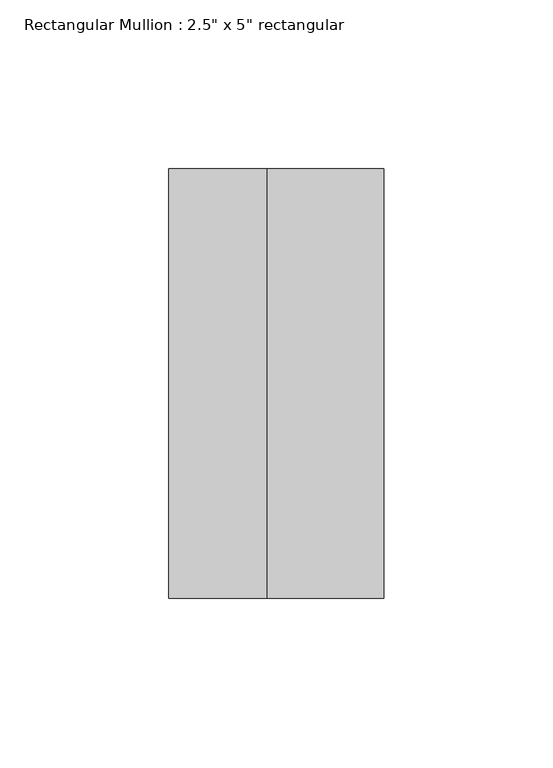
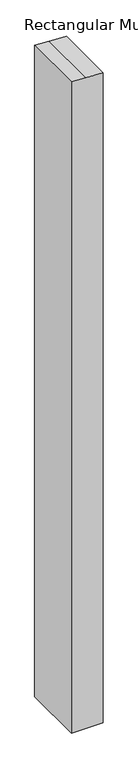
"""IFC4 building model written with IfcOpenShell, lengths in millimetres: member geometry."""

import ifcopenshell
import ifcopenshell.guid

model = None  # the IFC model being written
_history = None  # IfcOwnerHistory: only IFC2X3 demands one
_inside = {}  # id of a spatial element -> (the spatial element, [elements in it])
_under = {}  # id of a project, library or spatial element -> (it, [spatial elements below it])
_declared = {}  # id of a project -> (the project, [libraries it declares])
_typed = {}  # id of a type object -> (the type object, [elements of that type])
_made_of = {}  # id of a material, layer set ... -> (it, [elements and type objects made of it])


def new_model(schema):
    """Start an empty IFC model of exactly this schema.

    Asked for "IFC4X3", IfcOpenShell would pick the latest addendum, in which some entities
    have other attributes; the version numbers below select the first issue.
    IFC2X3 requires an IfcOwnerHistory on every rooted entity: one is made here for all.
    """
    global model, _history
    if schema == "IFC4X3":
        model = ifcopenshell.file(schema_version=(4, 3, 0, 0))
    else:
        model = ifcopenshell.file(schema=schema)
    _inside.clear()
    _under.clear()
    _declared.clear()
    _typed.clear()
    _made_of.clear()
    _history = None
    if model.schema == "IFC2X3":
        org = make("IfcOrganization", Name="unknown")
        user = make(
            "IfcPersonAndOrganization",
            ThePerson=make("IfcPerson", FamilyName="unknown"),
            TheOrganization=org,
        )
        app = make(
            "IfcApplication",
            ApplicationDeveloper=org,
            Version="unknown",
            ApplicationFullName="unknown",
            ApplicationIdentifier="unknown",
        )
        _history = make(
            "IfcOwnerHistory",
            OwningUser=user,
            OwningApplication=app,
            ChangeAction="ADDED",
            CreationDate=0,
        )
    return model


def make(cls, **values):
    """One entity of the class cls with the attributes given. An attribute that is None is left unset."""
    return model.create_entity(
        cls, **{name: value for name, value in values.items() if value is not None}
    )


def rooted(cls, **values):
    """An entity with a GlobalId (a new one), such as an element, a storey or a relation."""
    return make(cls, GlobalId=ifcopenshell.guid.new(), OwnerHistory=_history, **values)


def si_unit(unit_type, name, prefix=None):
    """IfcSIUnit, for example si_unit("LENGTHUNIT", "METRE", prefix="MILLI")."""
    return make("IfcSIUnit", UnitType=unit_type, Prefix=prefix, Name=name)


def assignment(units):
    """IfcUnitAssignment: the units of a project."""
    return None if units is None else make("IfcUnitAssignment", Units=units)


def point(xyz):
    """IfcCartesianPoint."""
    return None if xyz is None else make("IfcCartesianPoint", Coordinates=xyz)


def direction(xyz):
    """IfcDirection."""
    return None if xyz is None else make("IfcDirection", DirectionRatios=xyz)


def frame(location, z_axis=None, x_axis=None):
    """IfcAxis2Placement3D, a coordinate frame: its origin and axes. An axis left out is left unset."""
    return make(
        "IfcAxis2Placement3D",
        Location=point(location),
        Axis=direction(z_axis),
        RefDirection=direction(x_axis),
    )


def origin():
    """The frame at (0, 0, 0) with its axes left unset."""
    return frame((0.0, 0.0, 0.0))


def place(relative_to, where):
    """IfcLocalPlacement: puts the frame where relative to a parent placement (None: the world)."""
    return make(
        "IfcLocalPlacement", PlacementRelTo=relative_to, RelativePlacement=where
    )


def context(
    kind, dimensions, precision=None, world=None, true_north=None, identifier=None
):
    """IfcGeometricRepresentationContext, for example the 3D "Model" context."""
    return make(
        "IfcGeometricRepresentationContext",
        ContextIdentifier=identifier,
        ContextType=kind,
        CoordinateSpaceDimension=dimensions,
        Precision=precision,
        WorldCoordinateSystem=world,
        TrueNorth=true_north,
    )


def project(units=None, contexts=None):
    """IfcProject with its units and contexts."""
    return rooted(
        "IfcProject",
        Name="project",
        RepresentationContexts=contexts,
        UnitsInContext=assignment(units),
    )


def spatial(cls, under=None, at=None, **own):
    """A site, building, storey or space (cls), placed at a placement, below another one or the project."""
    s = rooted(cls, ObjectPlacement=at, **own)
    if under is not None:
        _under.setdefault(under.id(), (under, []))[1].append(s)
    return s


def polyline(points):
    """IfcPolyline through the points."""
    return make("IfcPolyline", Points=[point(p) for p in points])


def outline(outer, holes=None, kind="AREA"):
    """IfcArbitraryClosedProfileDef: a profile drawn as a closed curve; with holes, ...WithVoids."""
    if holes is None:
        return make("IfcArbitraryClosedProfileDef", ProfileType=kind, OuterCurve=outer)
    return make(
        "IfcArbitraryProfileDefWithVoids",
        ProfileType=kind,
        OuterCurve=outer,
        InnerCurves=holes,
    )


def extrude(swept, where, along, depth):
    """IfcExtrudedAreaSolid: the profile swept, set in the frame where, extruded along a direction by depth."""
    return make(
        "IfcExtrudedAreaSolid",
        SweptArea=swept,
        Position=where,
        ExtrudedDirection=direction(along),
        Depth=depth,
    )


def shape(context_of_items, identifier, shape_type, items):
    """IfcShapeRepresentation: the items that make up one representation, for example the "Body"."""
    return make(
        "IfcShapeRepresentation",
        ContextOfItems=context_of_items,
        RepresentationIdentifier=identifier,
        RepresentationType=shape_type,
        Items=items,
    )


def source(mapping_origin, context_of_items, identifier, shape_type, items):
    """IfcRepresentationMap: a shape defined once, which mapped items show again and again."""
    return make(
        "IfcRepresentationMap",
        MappingOrigin=mapping_origin,
        MappedRepresentation=shape(context_of_items, identifier, shape_type, items),
    )


def transform(
    local_origin,
    x_axis=None,
    y_axis=None,
    z_axis=None,
    scale=None,
    scale2=None,
    scale3=None,
    uniform=True,
):
    """IfcCartesianTransformationOperator3D, or its non-uniform kind. x_axis, y_axis, z_axis: its Axis1, 2, 3."""
    if uniform:
        return make(
            "IfcCartesianTransformationOperator3D",
            Axis1=direction(x_axis),
            Axis2=direction(y_axis),
            LocalOrigin=point(local_origin),
            Scale=scale,
            Axis3=direction(z_axis),
        )
    return make(
        "IfcCartesianTransformationOperator3DnonUniform",
        Axis1=direction(x_axis),
        Axis2=direction(y_axis),
        LocalOrigin=point(local_origin),
        Scale=scale,
        Axis3=direction(z_axis),
        Scale2=scale2,
        Scale3=scale3,
    )


def mapped(mapping_source, mapping_target):
    """IfcMappedItem: shows the shape of a source again, moved by a transform."""
    return make(
        "IfcMappedItem", MappingSource=mapping_source, MappingTarget=mapping_target
    )


def made_of(thing, what):
    """Note that an element or type object is made of a material, layer set ...; save() writes the relation."""
    if what is not None:
        _made_of.setdefault(what.id(), (what, []))[1].append(thing)
    return thing


def element(
    cls,
    number,
    at=None,
    inside=None,
    cuts=None,
    type_object=None,
    material=None,
    context=None,
    identifier="Body",
    shape_type=None,
    held_by="IfcProductDefinitionShape",
    body=None,
    shapes=None,
    **own,
):
    """One element of the class cls, such as IfcWall. Its Tag is "e" and its number.

    at: its placement. inside: the storey or other place that contains it. cuts: it is an
    opening in that element (IfcRelVoidsElement). A single representation is given by context,
    identifier, shape_type and body (its items); several are given by shapes. held_by: the class
    of the entity that holds the representations. save() writes the other relations.
    """
    e = rooted(cls, Tag="e%d" % number, ObjectPlacement=at, **own)
    if body is not None:
        shapes = [shape(context, identifier, shape_type, body)]
    if shapes is not None:
        e.Representation = make(held_by, Representations=shapes)
    if inside is not None:
        _inside.setdefault(inside.id(), (inside, []))[1].append(e)
    if cuts is not None:
        rooted(
            "IfcRelVoidsElement", RelatingBuildingElement=cuts, RelatedOpeningElement=e
        )
    if type_object is not None:
        _typed.setdefault(type_object.id(), (type_object, []))[1].append(e)
    return made_of(e, material)


def aggregate(whole, parts):
    """IfcRelAggregates: a whole, such as a stair, and the parts it consists of."""
    return rooted("IfcRelAggregates", RelatingObject=whole, RelatedObjects=parts)


def save(model, path):
    """Write the relations noted so far, then the file.

    IfcRelAggregates (storeys below a building ...), IfcRelContainedInSpatialStructure (elements
    in a storey), IfcRelDefinesByType, IfcRelAssociatesMaterial and IfcRelDeclares: one each for
    every whole, place, type object, material and project.
    """
    for whole, parts in _under.values():
        aggregate(whole, parts)
    for where, things in _inside.values():
        rooted(
            "IfcRelContainedInSpatialStructure",
            RelatedElements=things,
            RelatingStructure=where,
        )
    for kind, things in _typed.values():
        rooted("IfcRelDefinesByType", RelatedObjects=things, RelatingType=kind)
    for what, things in _made_of.values():
        rooted("IfcRelAssociatesMaterial", RelatedObjects=things, RelatingMaterial=what)
    for by, libraries in _declared.values():
        rooted("IfcRelDeclares", RelatingContext=by, RelatedDefinitions=libraries)
    model.write(path)


def member_2c70c373(model_context):
    return source(origin(), model_context, "Body", "SweptSolid", [
        extrude(outline(polyline([(-64.8775557, 31.75), (-63.4449853, -2.6426951), (-62.232569, -31.75), (-1437.7204901, -31.75), (-1437.7204901, 31.75), (-64.8775557, 31.75)])), frame((0.0, -63.5, 0.0), z_axis=(0.0, 1.0, 0.0), x_axis=(0.0, 0.0, 1.0)), (0.0, 0.0, 1.0), 127.0),
    ])


if __name__ == "__main__":
    model = new_model("IFC4")
    model_context = context("Model", 3, world=origin())
    ifc_project = project(units=[si_unit("LENGTHUNIT", "METRE", prefix="MILLI")], contexts=[model_context])
    site = spatial("IfcSite", under=ifc_project)
    building = spatial("IfcBuilding", under=site)
    placement = place(None, origin())
    member_shape = member_2c70c373(model_context)
    element("IfcMember", 1, ObjectType="Rectangular Mullion : 2.5\" x 5\" rectangular", at=placement, inside=building, context=model_context, shape_type="MappedRepresentation", body=[
        mapped(member_shape, transform((0.0, 0.0, 0.0), x_axis=(1.0, 0.0, 0.0), y_axis=(0.0, 1.0, 0.0), z_axis=(0.0, 0.0, 1.0))),
    ])
    save(model, "model.ifc")

# Revit data of these elements
# Type "Rectangular Mullion : 2.5\" x 5\" rectangular"
#   built-in parameter 1007304 = 0.416667 (stored number, unit not read)
#   built-in parameter 1007301 = 0.104167 (stored number, unit not read)
#   built-in parameter 1007300 = 0.104167 (stored number, unit not read)
# Element 1 (IfcMember, "Rectangular Mullion : 2.5\" x 5\" rectangular")
#   Materials on its faces: "Aluminum"
# Materials
#   "Aluminum": class "Metal", colour RGB 247 247 247, transparency 0, Description = "Aluminum 6061", Cost = 0
